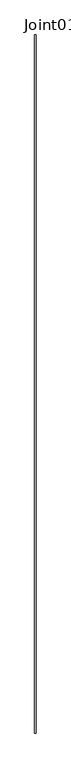
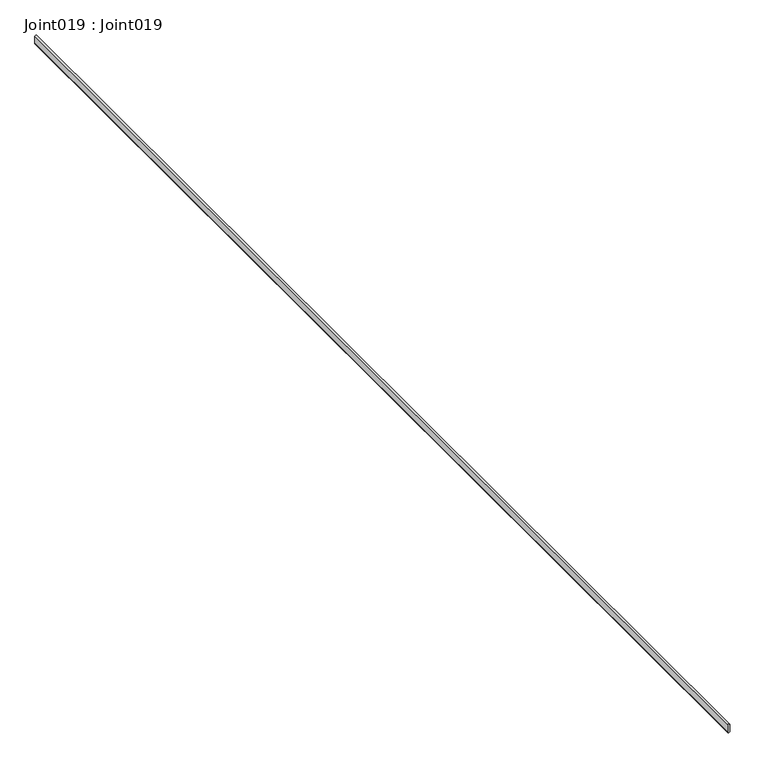
"""IFC4 building model written with IfcOpenShell, lengths in millimetres: proxy geometry, Joint019 : Joint019."""

from ifc_helpers import new_model, si_unit, point, frame, frame_2d, origin, place, context, project, spatial, polyline, circle_curve, trimmed, segment, composite_curve, outline, extrude, source, transform, mapped, element, save


def joint019_joint019_3ecd68ab(model_context):
    return source(origin(), model_context, "Body", "SweptSolid", [
        extrude(outline(composite_curve([segment(polyline([(43045.6850385, -6491.4926763), (43033.6103315, -6491.4926763)]), True, "CONTINUOUS"), segment(trimmed(circle_curve(frame_2d((43033.6103315, -6489.7270513)), 1.765625), [point((43033.6103315, -6491.4926763))], [point((43033.6103315, -6487.9614263))], False, "CARTESIAN"), True, "CONTINUOUS"), segment(polyline([(43033.6103315, -6487.9614263), (43045.6850385, -6487.9614263)]), True, "CONTINUOUS"), segment(trimmed(circle_curve(frame_2d((43045.6850385, -6489.7270513)), 1.765625), [point((43045.6850385, -6487.9614263))], [point((43045.6850385, -6491.4926763))], False, "CARTESIAN"), True, "CONTINUOUS")], self_intersect=False)), frame((0.0, 7982.1531721, 0.0), z_axis=(0.0, 1.0, 0.0), x_axis=(0.0, 0.0, 1.0)), (0.0, 0.0, 1.0), 2000.0),
    ])


if __name__ == "__main__":
    model = new_model("IFC4")
    model_context = context("Model", 3, world=origin())
    ifc_project = project(units=[si_unit("LENGTHUNIT", "METRE", prefix="MILLI")], contexts=[model_context])
    site = spatial("IfcSite", under=ifc_project)
    building = spatial("IfcBuilding", under=site)
    placement = place(None, origin())
    joint019_joint019_shape = joint019_joint019_3ecd68ab(model_context)
    element("IfcBuildingElementProxy", 1, Name="Joint019 : Joint019", ObjectType="Joint019 : Joint019", at=placement, inside=building, context=model_context, shape_type="MappedRepresentation", body=[
        mapped(joint019_joint019_shape, transform((0.0, 0.0, 0.0), x_axis=(1.0, 0.0, 0.0), y_axis=(0.0, 1.0, 0.0), z_axis=(0.0, 0.0, 1.0))),
    ])
    save(model, "model.ifc")

# Revit data of these elements
# Type "Joint019 : Joint019"
#   NameOverride = "Joint019"
# Element 1 (IfcBuildingElementProxy, "Joint019 : Joint019")
#   Materials on its faces: "SILICON JOINT"
# Materials
#   "SILICON JOINT": class "Unassigned", colour RGB 150 184 127, transparency 0
